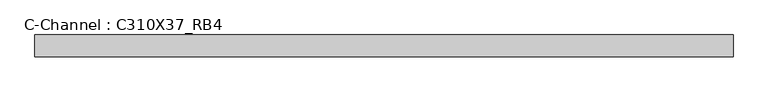
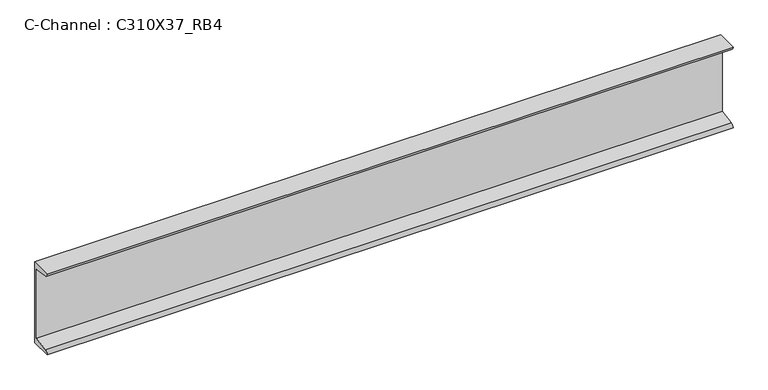
"""IFC4 building model written with IfcOpenShell, lengths in millimetres: beam geometry, C-Channel : C310X37_RB4."""

from ifc_helpers import new_model, si_unit, point, frame, frame_2d, origin, place, context, project, spatial, polyline, circle_curve, trimmed, segment, composite_curve, outline, extrude, source, transform, mapped, element, save


def c_channel_c310x37_rb4_80b00117(model_context):
    return source(origin(), model_context, "Body", "SweptSolid", [
        extrude(outline(composite_curve([segment(polyline([(17.1196, 152.4), (17.1196, -152.4), (-60.3504, -152.4)]), True, "CONTINUOUS"), segment(trimmed(circle_curve(frame_2d((-47.625, -152.4)), 12.7254), [point((-60.3504, -152.4))], [point((-47.625, -139.6746))], False, "CARTESIAN"), True, "CONTINUOUS"), segment(polyline([(-47.625, -139.6746), (7.2898, -130.9769501), (7.2898, 130.9769501), (-47.625, 139.6746)]), True, "CONTINUOUS"), segment(trimmed(circle_curve(frame_2d((-47.625, 152.4)), 12.7254), [point((-47.625, 139.6746))], [point((-60.3504, 152.4))], False, "CARTESIAN"), True, "CONTINUOUS"), segment(polyline([(-60.3504, 152.4), (17.1196, 152.4)]), True, "CONTINUOUS")], self_intersect=False)), frame((-1279.1307311, 0.0, 0.0), z_axis=(1.0, 0.0, 0.0), x_axis=(0.0, 1.0, 0.0)), (0.0, 0.0, 1.0), 2452.8723053),
    ])


if __name__ == "__main__":
    model = new_model("IFC4")
    model_context = context("Model", 3, world=origin())
    ifc_project = project(units=[si_unit("LENGTHUNIT", "METRE", prefix="MILLI")], contexts=[model_context])
    site = spatial("IfcSite", under=ifc_project)
    building = spatial("IfcBuilding", under=site)
    placement = place(None, origin())
    c_channel_c310x37_rb4_shape = c_channel_c310x37_rb4_80b00117(model_context)
    element("IfcBeam", 1, ObjectType="C-Channel : C310X37_RB4", at=placement, inside=building, context=model_context, shape_type="MappedRepresentation", body=[
        mapped(c_channel_c310x37_rb4_shape, transform((0.0, 0.0, 0.0), x_axis=(1.0, 0.0, 0.0), y_axis=(0.0, 1.0, 0.0), z_axis=(0.0, 0.0, 1.0))),
    ])
    save(model, "model.ifc")

# Revit data of these elements
# Type "C-Channel : C310X37_RB4"
#   Assembly Code = "B10"
#   W = 25
#   Length [instance default] = 1524 mm
#   bf = 77.47 mm
#   d = 304.8 mm
#   tf = 12.725 mm
#   tw = 9.83 mm
#   x = 17.12 mm
#   A = 0.00473547 m²
#   Structural Material [instance default] = Steel ASTM A36
# Element 1 (IfcBeam, "C-Channel : C310X37_RB4")
#   Structural Material = Steel ASTM A992
#   Materials on its faces: "Steel ASTM A992"
# Materials
#   "Steel ASTM A36": class "Metal", colour RGB 199 199 199, transparency 0, Description = "Structural steel, ASTM A36 Grade B, mill finish", Cost = 0
#   "Steel ASTM A992": class "Metal", colour RGB 199 199 199, transparency 0, Description = "Structural steel 50ksi", Cost = 0
